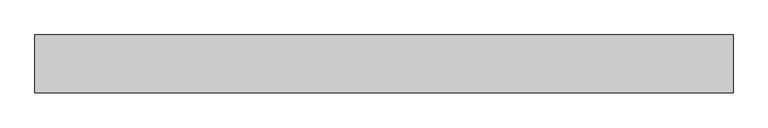
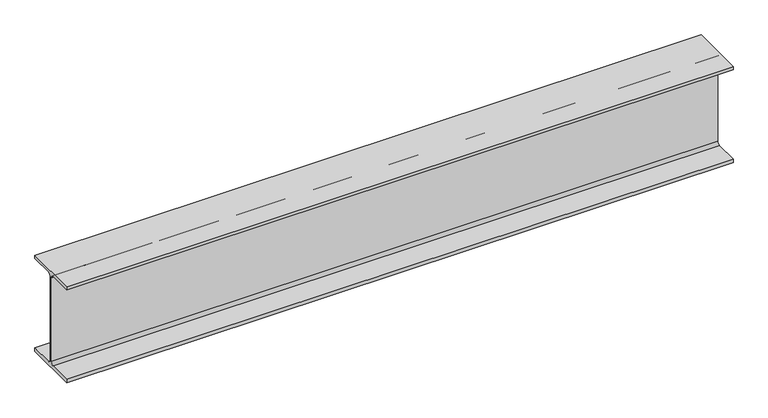
"""IFC4 building model written with IfcOpenShell, lengths in millimetres: beam geometry, Old_Steel Beam_H-KSD3502 : H_SB_ASB_H-200×200x8x12."""

from ifc_helpers import new_model, si_unit, point, frame, frame_2d, origin, place, context, project, spatial, polyline, circle_curve, trimmed, segment, composite_curve, outline, extrude, source, transform, mapped, element, save


def beam_169b0a2c(model_context):
    return source(origin(), model_context, "Body", "SweptSolid", [
        extrude(outline(composite_curve([segment(polyline([(82.5, -141.5), (82.5, -151.7), (-82.5, -151.7), (-82.5, -141.5), (-11.9, -141.5)]), True, "CONTINUOUS"), segment(trimmed(circle_curve(frame_2d((-11.9, -132.6)), 8.9), [point((-11.9, -141.5))], [point((-3.0, -132.6))], True, "CARTESIAN"), True, "CONTINUOUS"), segment(polyline([(-3.0, -132.6), (-3.0, 132.6)]), True, "CONTINUOUS"), segment(trimmed(circle_curve(frame_2d((-11.9, 132.6)), 8.9), [point((-3.0, 132.6))], [point((-11.9, 141.5))], True, "CARTESIAN"), True, "CONTINUOUS"), segment(polyline([(-11.9, 141.5), (-82.5, 141.5), (-82.5, 151.7), (82.5, 151.7), (82.5, 141.5), (11.9, 141.5)]), True, "CONTINUOUS"), segment(trimmed(circle_curve(frame_2d((11.9, 132.6)), 8.9), [point((11.9, 141.5))], [point((3.0, 132.6))], True, "CARTESIAN"), True, "CONTINUOUS"), segment(polyline([(3.0, 132.6), (3.0, -132.6)]), True, "CONTINUOUS"), segment(trimmed(circle_curve(frame_2d((11.9, -132.6)), 8.9), [point((3.0, -132.6))], [point((11.9, -141.5))], True, "CARTESIAN"), True, "CONTINUOUS"), segment(polyline([(11.9, -141.5), (82.5, -141.5)]), True, "CONTINUOUS")], self_intersect=False)), frame((-1045.4188164, 0.0, 0.0), z_axis=(1.0, 0.0, 0.0), x_axis=(0.0, 1.0, 0.0)), (0.0, 0.0, 1.0), 1992.0019459),
    ])


if __name__ == "__main__":
    model = new_model("IFC4")
    model_context = context("Model", 3, world=origin())
    ifc_project = project(units=[si_unit("LENGTHUNIT", "METRE", prefix="MILLI")], contexts=[model_context])
    site = spatial("IfcSite", under=ifc_project)
    building = spatial("IfcBuilding", under=site)
    placement = place(None, origin())
    beam_shape = beam_169b0a2c(model_context)
    element("IfcBeam", 1, ObjectType="Old_Steel Beam_H-KSD3502 : H_SB_ASB_H-200×200x8x12", at=placement, inside=building, context=model_context, shape_type="MappedRepresentation", body=[
        mapped(beam_shape, transform((0.0, 0.0, 0.0), x_axis=(1.0, 0.0, 0.0), y_axis=(0.0, 1.0, 0.0), z_axis=(0.0, 0.0, 1.0))),
    ])
    save(model, "model.ifc")

# Revit data of these elements
# Type "Old_Steel Beam_H-KSD3502 : H_SB_ASB_H-200×200x8x12"
#   Width = 20.0 cm
#   Web Thickness = 0.8 cm
#   Web Fillet = 1.3 cm
#   Warping Constant = 141376.0 cm⁶
#   Torsional Moment of Inertia = 26.2485 cm⁴
#   Torsional Modulus = 1.0 cm³
#   Section Area = 63.53 cm²
#   Plastic Modulus weak axis = 244.0 cm³
#   Plastic Modulus strong axis = 525.0 cm³
#   Perimeter = 1.16 m²/m
#   Nominal Weight = 49.90 kgf/m
#   Moment of Inertia weak axis = 1600.00 cm⁴
#   Moment of Inertia strong axis = 4720.00 cm⁴
#   Height = 20.0 cm
#   Flange Thickness = 1.2 cm
#   Elastic Modulus weak axis = 160.0 cm³
#   Elastic Modulus strong axis = 472.0 cm³
#   Centroid Vertical = 10.0 cm
#   Centroid Horizontal = 10.0 cm
#   Length [instance default] = 1.5240 m
#   Structural Material [instance default] = Steel, 45-345
#   Assembly Code = ""
# Element 1 (IfcBeam, "Old_Steel Beam_H-KSD3502 : H_SB_ASB_H-200×200x8x12")
#   Structural Material = none
# Materials
#   "Steel, 45-345": class "Metal", colour RGB 189 187 185, transparency 0, Description = "Steel 345 MPa", Cost = 0
